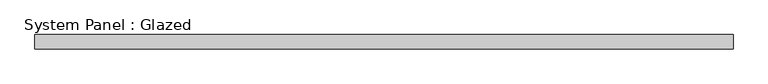
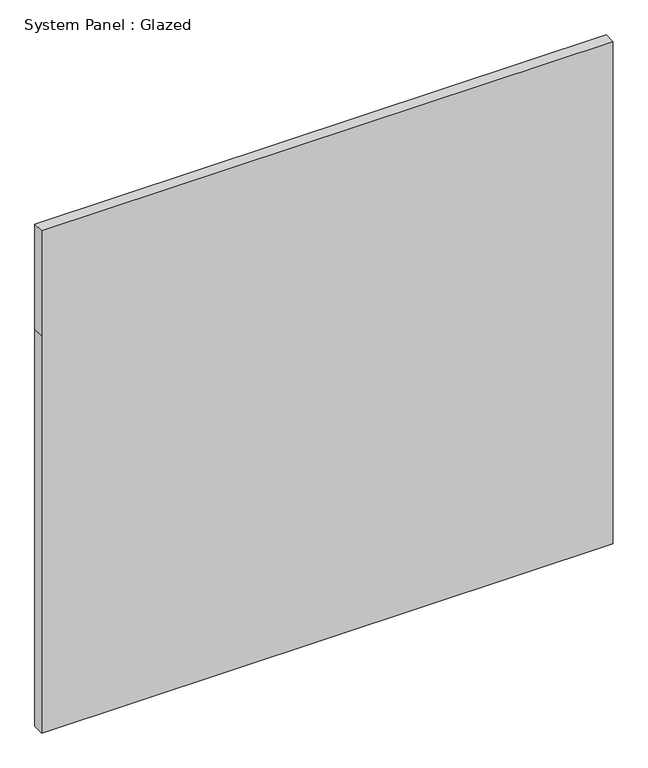
"""IFC4 building model written with IfcOpenShell, lengths in millimetres: plate geometry, System Panel : Glazed."""

from ifc_helpers import new_model, si_unit, frame, origin, place, context, project, spatial, polyline, outline, extrude, source, transform, mapped, element, save


def system_panel_glazed_ea10912d(model_context):
    return source(origin(), model_context, "Body", "SweptSolid", [
        extrude(outline(polyline([(0.0, -622.3), (0.0, 622.3), (914.4, 622.3), (1155.7, 622.3), (1155.7, -622.3), (914.4, -622.3), (0.0, -622.3)])), frame((0.0, 19.05, 0.0), z_axis=(0.0, 1.0, 0.0), x_axis=(0.0, 0.0, 1.0)), (0.0, 0.0, 1.0), 25.4),
    ])


if __name__ == "__main__":
    model = new_model("IFC4")
    model_context = context("Model", 3, world=origin())
    ifc_project = project(units=[si_unit("LENGTHUNIT", "METRE", prefix="MILLI")], contexts=[model_context])
    site = spatial("IfcSite", under=ifc_project)
    building = spatial("IfcBuilding", under=site)
    placement = place(None, origin())
    system_panel_glazed_shape = system_panel_glazed_ea10912d(model_context)
    element("IfcPlate", 1, ObjectType="System Panel : Glazed", at=placement, inside=building, context=model_context, shape_type="MappedRepresentation", body=[
        mapped(system_panel_glazed_shape, transform((0.0, 0.0, 0.0), x_axis=(1.0, 0.0, 0.0), y_axis=(0.0, 1.0, 0.0), z_axis=(0.0, 0.0, 1.0))),
    ])
    save(model, "model.ifc")

# Revit data of these elements
# Element 1 (IfcPlate, "System Panel : Glazed")
#   Materials on its faces: "Glass"
# Materials
#   "Glass": class "Glass", colour RGB 0 128 192, transparency 0.75
